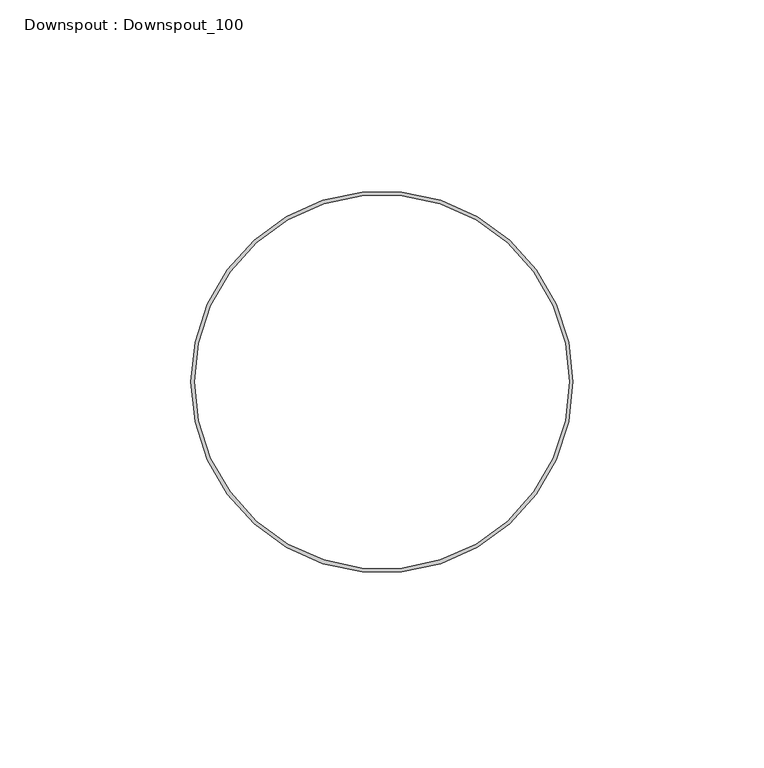
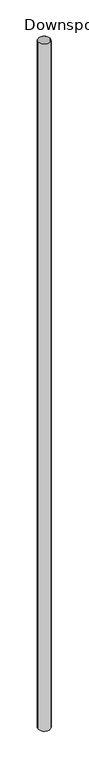
"""IFC4 building model written with IfcOpenShell, lengths in millimetres: proxy geometry, Downspout : Downspout_100."""

from ifc_helpers import new_model, si_unit, point, origin, origin_with_axes, origin_2d, place, context, project, spatial, circle_curve, trimmed, segment, composite_curve, outline, extrude, source, transform, mapped, element, save


def downspout_downspout_100_a2d51f41(model_context):
    return source(origin(), model_context, "Body", "SweptSolid", [
        extrude(outline(composite_curve([segment(trimmed(circle_curve(origin_2d(), 50.0), [point((50.0, 0.0))], [point((-50.0, 0.0))], False, "CARTESIAN"), True, "CONTINUOUS"), segment(trimmed(circle_curve(origin_2d(), 50.0), [point((-50.0, 0.0))], [point((50.0, 0.0))], False, "CARTESIAN"), True, "CONTINUOUS")], self_intersect=False), holes=[composite_curve([segment(trimmed(circle_curve(origin_2d(), 49.0), [point((49.0, 0.0))], [point((-49.0, 0.0))], True, "CARTESIAN"), True, "CONTINUOUS"), segment(trimmed(circle_curve(origin_2d(), 49.0), [point((-49.0, 0.0))], [point((49.0, 0.0))], True, "CARTESIAN"), True, "CONTINUOUS")], self_intersect=False)]), origin_with_axes(), (0.0, 0.0, 1.0), 6100.0),
    ])


if __name__ == "__main__":
    model = new_model("IFC4")
    model_context = context("Model", 3, world=origin())
    ifc_project = project(units=[si_unit("LENGTHUNIT", "METRE", prefix="MILLI")], contexts=[model_context])
    site = spatial("IfcSite", under=ifc_project)
    building = spatial("IfcBuilding", under=site)
    placement = place(None, origin())
    downspout_downspout_100_shape = downspout_downspout_100_a2d51f41(model_context)
    element("IfcBuildingElementProxy", 1, Name="Downspout : Downspout_100", ObjectType="Downspout : Downspout_100", at=placement, inside=building, context=model_context, shape_type="MappedRepresentation", body=[
        mapped(downspout_downspout_100_shape, transform((0.0, 0.0, 0.0), x_axis=(1.0, 0.0, 0.0), y_axis=(0.0, 1.0, 0.0), z_axis=(0.0, 0.0, 1.0))),
    ])
    save(model, "model.ifc")

# Revit data of these elements
# Type "Downspout : Downspout_100"
#   Thickness = 2 mm
#   Diameter(Inner) = 98 mm
#   Diameter = 100 mm
#   hec_material3 [instance default] = none
#   hec_material2 [instance default] = none
#   hec_material1 [instance default] = none
#   Structural Material [instance default] = none
#   Default Elevation = 0
# Element 1 (IfcBuildingElementProxy, "Downspout : Downspout_100")
#   hec_material2 = A04AU175-00001_Splash Block_Precast Conc Block
#   hec_material1 = A04AU174-00001_Water Collection Box_Galv. Steel Type
#   Structural Material = A04AU173-00001_Downspout_Galv. Steel Type_D100
#   Materials on its faces: "A04AU173-00001_Downspout_Galv. Steel Type_D100"
# Materials
#   "A04AU173-00001_Downspout_Galv. Steel Type_D100": class "Metal", colour RGB 148 148 148, transparency 0, Description = "Steel", W00) Work Master Code = "A04AU173-00001", W01) Work Master_Lv1 = "Finishing Work", W02) Work Master_Lv2 = "Misc. Work", W03) Work Master_Spec.1 = "Downspout", W04) Work Master_Spec.2 = "Galvanized Steel Type", W05) Work Master_Spec.3 = "w/ Fixing Accessories", W06) Work Master_Spec.4 = "DIA=100mm", Cost = 0
#   "A04AU175-00001_Splash Block_Precast Conc Block": class "Concrete", colour RGB 115 116 108, transparency 0, Description = "Precast concrete", W00) Work Master Code = "A04AU175-00001", W01) Work Master_Lv1 = "Finishing Work", W02) Work Master_Lv2 = "Misc. Work", W03) Work Master_Spec.1 = "Splash Block", W04) Work Master_Spec.2 = "Precast Concrete Block Type", Cost = 0
#   "A04AU174-00001_Water Collection Box_Galv. Steel Type": class "Metal", colour RGB 148 148 148, transparency 0, Description = "Steel", W00) Work Master Code = "A04AU174-00001", W01) Work Master_Lv1 = "Finishing Work", W02) Work Master_Lv2 = "Misc. Work", W03) Work Master_Spec.1 = "Water Collection Box", W04) Work Master_Spec.2 = "Galvanized Steel Type", W05) Work Master_Spec.3 = "w/ Fixing Accessories", Cost = 0
